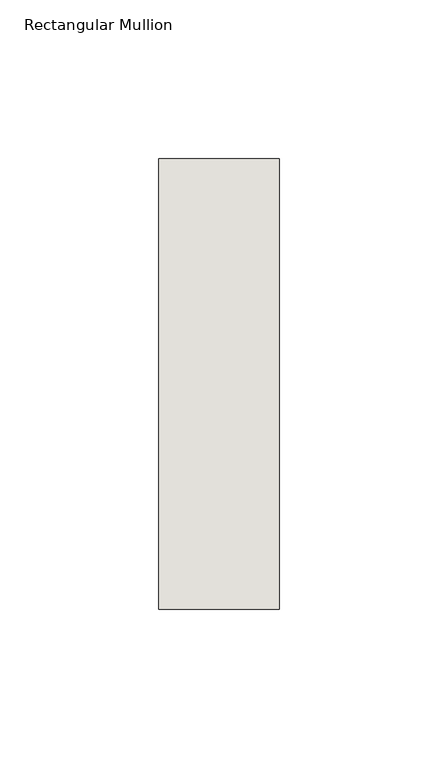
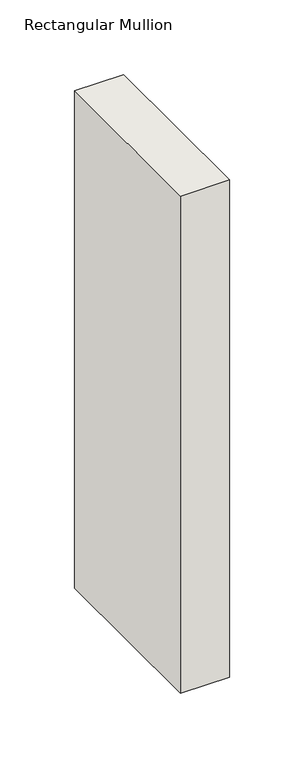
"""IFC4 building model written with IfcOpenShell, lengths in millimetres: wall geometry, Rectangular Mullion : NLRS_21_CWM_hsb-regel 38x142_gen_rsf."""

from ifc_helpers import new_model, si_unit, frame, origin, place, context, project, spatial, polyline, outline, extrude, source, transform, mapped, element, save


def rectangular_mullion_e91dba32(model_context):
    return source(origin(), model_context, "Body", "SweptSolid", [
        extrude(outline(polyline([(19.0, -71.0), (-19.0, -71.0), (-19.0, 71.0), (19.0, 71.0), (19.0, -71.0)])), frame((0.0, 0.0, -407.0), z_axis=(0.0, 0.0, 1.0), x_axis=(1.0, 0.0, 0.0)), (0.0, 0.0, 1.0), 407.0),
    ])


if __name__ == "__main__":
    model = new_model("IFC4")
    model_context = context("Model", 3, world=origin())
    ifc_project = project(units=[si_unit("LENGTHUNIT", "METRE", prefix="MILLI")], contexts=[model_context])
    site = spatial("IfcSite", under=ifc_project)
    building = spatial("IfcBuilding", under=site)
    placement = place(None, origin())
    rectangular_mullion_shape = rectangular_mullion_e91dba32(model_context)
    element("IfcWall", 1, ObjectType="Rectangular Mullion : NLRS_21_CWM_hsb-regel 38x142_gen_rsf", at=placement, inside=building, context=model_context, shape_type="MappedRepresentation", body=[
        mapped(rectangular_mullion_shape, transform((0.0, 0.0, 0.0), x_axis=(1.0, 0.0, 0.0), y_axis=(0.0, 1.0, 0.0), z_axis=(0.0, 0.0, 1.0))),
    ])
    save(model, "model.ifc")

# Revit data of these elements
# Type "Rectangular Mullion : NLRS_21_CWM_hsb-regel 38x142_gen_rsf"
#   Type IfcGUID = "07M7mRoiH1CR8m_RSKIwpF"
#   Assembly Code = "21.10"
#   IfcExportAs = "IfcWall"
#   built-in parameter 1007322 = 0.465879 (stored number, unit not read)
#   built-in parameter 1007321 = 0.062336 (stored number, unit not read)
#   built-in parameter 1007320 = 0.062336 (stored number, unit not read)
# Element 1 (IfcWall, "Rectangular Mullion : NLRS_21_CWM_hsb-regel 38x142_gen_rsf")
#   Materials on its faces: "NLRS_i2_hout naaldhout vuren_gen_rsf"
# Materials
#   "NLRS_i2_hout naaldhout vuren_gen_rsf": class "I - Hout", colour RGB 234 199 147, transparency 0, Keynote = "i2", Manufacturer = "Revit Standards Foundation", URL = "www.revitstandards.org", Description = "hout vuren", Cost = 0
